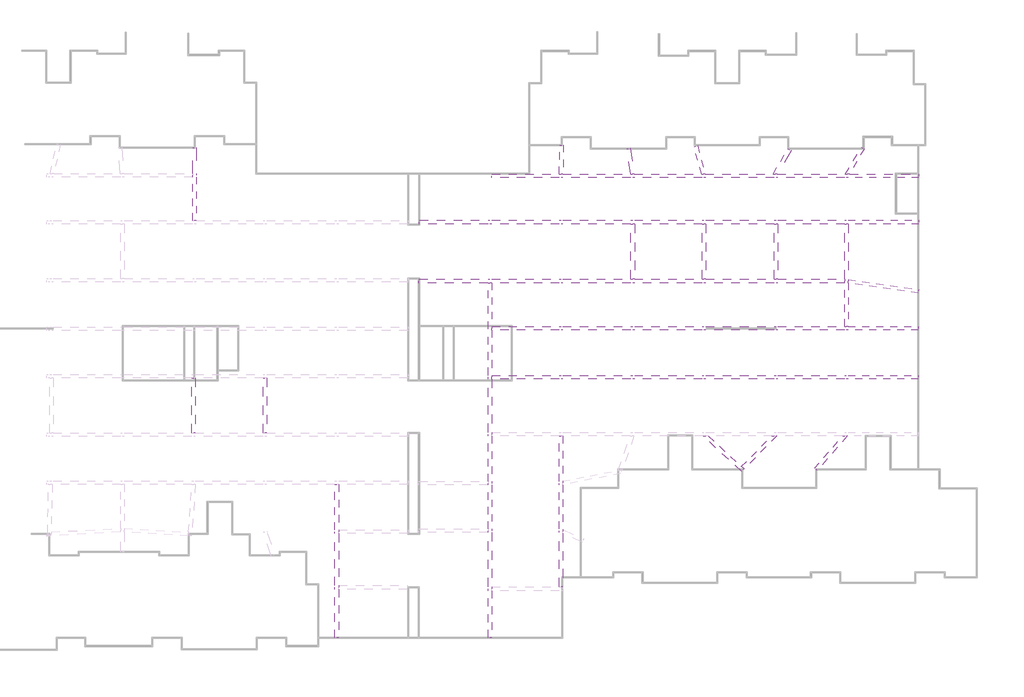
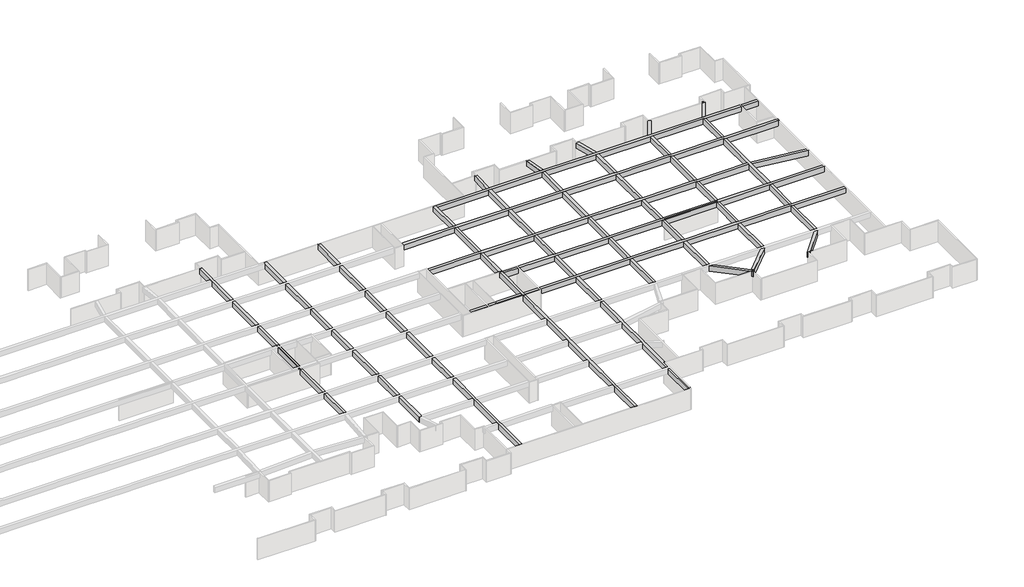
# One storey, part 16 of 16: 24 beams.
"""IFC4 building model written with IfcOpenShell, lengths in millimetres."""

from ifc_helpers import new_model, si_unit, frame, origin, place, context, project, spatial, polyline, outline, extrude, faceted_brep, element, save

model = new_model("IFC4")

# Units and contexts
model_context = context("Model", 3, world=origin())
ifc_project = project(units=[si_unit("LENGTHUNIT", "METRE", prefix="MILLI")], contexts=[model_context])

# Site, building, storey
site = spatial("IfcSite", under=ifc_project)
building = spatial("IfcBuilding", under=site)
storey = spatial("IfcBuildingStorey", under=building, Name="户型图", Elevation=0.0)

# Beams
placement = place(None, origin())
element("IfcBeam", 1, ObjectType="混凝土 - 矩形梁 : KL_beam", at=placement, inside=storey, context=model_context, shape_type="Brep", body=[
    faceted_brep([(470553.7576761, -137545.1471775, 3300.0), (470553.7576761, -137945.1471775, 3300.0), (470553.7576761, -137945.1471775, 2500.0), (470553.7576761, -137545.1471775, 2500.0), (414553.7576761, -137545.1471775, 3300.0), (414553.7576761, -137545.1471775, 2500.0), (414553.7576761, -137945.1471775, 2500.0), (414553.7576761, -137945.1471775, 3300.0), (462649.4319412, -137545.1471775, 3300.0), (462249.4319412, -137545.1471775, 3300.0), (454758.8748808, -137545.1471775, 3300.0), (454358.8748808, -137545.1471775, 3300.0), (446653.757676, -137545.1471775, 3300.0), (446253.757676, -137545.1471775, 3300.0), (438676.3481949, -137545.1471775, 3300.0), (438276.3481949, -137545.1471775, 3300.0), (430644.9716608, -137545.1471775, 3300.0), (430244.9716608, -137545.1471775, 3300.0), (422643.757676, -137545.1471775, 3300.0), (422243.757676, -137545.1471775, 3300.0), (422243.757676, -137945.1471775, 3300.0), (422643.757676, -137945.1471775, 3300.0), (430244.9716608, -137945.1471775, 3300.0), (430644.9716608, -137945.1471775, 3300.0), (438276.3481949, -137945.1471775, 3300.0), (438676.3481949, -137945.1471775, 3300.0), (446253.757676, -137945.1471775, 3300.0), (446653.757676, -137945.1471775, 3300.0), (454358.8748808, -137945.1471775, 3300.0), (454758.8748808, -137945.1471775, 3300.0), (462249.4319412, -137945.1471775, 3300.0), (462649.4319412, -137945.1471775, 3300.0), (422243.757676, -137945.1471775, 2500.0), (422643.757676, -137945.1471775, 2500.0), (430244.9716608, -137945.1471775, 2500.0), (430644.9716608, -137945.1471775, 2500.0), (438276.3481949, -137945.1471775, 2500.0), (438676.3481949, -137945.1471775, 2500.0), (446253.757676, -137945.1471775, 2500.0), (446653.757676, -137945.1471775, 2500.0), (454358.8748808, -137945.1471775, 2500.0), (454758.8748808, -137945.1471775, 2500.0), (462249.4319412, -137945.1471775, 2500.0), (462649.4319412, -137945.1471775, 2500.0), (422243.757676, -137545.1471775, 2500.0), (422643.757676, -137545.1471775, 2500.0), (430244.9716608, -137545.1471775, 2500.0), (430644.9716608, -137545.1471775, 2500.0), (438276.3481949, -137545.1471775, 2500.0), (438676.3481949, -137545.1471775, 2500.0), (446253.757676, -137545.1471775, 2500.0), (446653.757676, -137545.1471775, 2500.0), (454358.8748808, -137545.1471775, 2500.0), (454758.8748808, -137545.1471775, 2500.0), (462249.4319412, -137545.1471775, 2500.0), (462649.4319412, -137545.1471775, 2500.0)], [[[0, 1, 2, 3]], [[4, 5, 6, 7]], [[1, 0, 8, 9, 10, 11, 12, 13, 14, 15, 16, 17, 18, 19, 4, 7, 20, 21, 22, 23, 24, 25, 26, 27, 28, 29, 30, 31]], [[2, 1, 31, 30, 29, 28, 27, 26, 25, 24, 23, 22, 21, 20, 7, 6, 32, 33, 34, 35, 36, 37, 38, 39, 40, 41, 42, 43]], [[3, 2, 43, 42, 41, 40, 39, 38, 37, 36, 35, 34, 33, 32, 6, 5, 44, 45, 46, 47, 48, 49, 50, 51, 52, 53, 54, 55]], [[0, 3, 55, 54, 53, 52, 51, 50, 49, 48, 47, 46, 45, 44, 5, 4, 19, 18, 17, 16, 15, 14, 13, 12, 11, 10, 9, 8]]]),
])
element("IfcBeam", 2, ObjectType="混凝土 - 矩形梁 : KL_beam", at=placement, inside=storey, context=model_context, shape_type="Brep", body=[
    faceted_brep([(414504.0948086, -144165.1471774, 3300.0), (414504.0948086, -144165.1471774, 2500.0), (414504.0948086, -144565.1471774, 2500.0), (414504.0948086, -144565.1471774, 3300.0), (422243.757676, -144565.1471774, 3300.0), (422643.757676, -144565.1471774, 3300.0), (430244.9716608, -144565.1471774, 3300.0), (430644.9716608, -144565.1471774, 3300.0), (438276.3481949, -144565.1471774, 3300.0), (438676.3481949, -144565.1471774, 3300.0), (446253.757676, -144565.1471774, 3300.0), (446653.757676, -144565.1471774, 3300.0), (454358.8748808, -144565.1471774, 3300.0), (454758.8748808, -144565.1471774, 3300.0), (462249.4319412, -144565.1471774, 3300.0), (462249.4319412, -144165.1471774, 3300.0), (454758.8748808, -144165.1471774, 3300.0), (454358.8748808, -144165.1471774, 3300.0), (446653.757676, -144165.1471774, 3300.0), (446253.757676, -144165.1471774, 3300.0), (438676.3481949, -144165.1471774, 3300.0), (438276.3481949, -144165.1471774, 3300.0), (430644.9716608, -144165.1471774, 3300.0), (430244.9716608, -144165.1471774, 3300.0), (422643.757676, -144165.1471774, 3300.0), (422243.757676, -144165.1471774, 3300.0), (422243.757676, -144565.1471774, 2500.0), (422643.757676, -144565.1471774, 2500.0), (430244.9716608, -144565.1471774, 2500.0), (430644.9716608, -144565.1471774, 2500.0), (438276.3481949, -144565.1471774, 2500.0), (438676.3481949, -144565.1471774, 2500.0), (446253.757676, -144565.1471774, 2500.0), (446653.757676, -144565.1471774, 2500.0), (454358.8748808, -144565.1471774, 2500.0), (454758.8748808, -144565.1471774, 2500.0), (462249.4319412, -144565.1471774, 2500.0), (422243.757676, -144165.1471774, 2500.0), (422643.757676, -144165.1471774, 2500.0), (430244.9716608, -144165.1471774, 2500.0), (430644.9716608, -144165.1471774, 2500.0), (438276.3481949, -144165.1471774, 2500.0), (438676.3481949, -144165.1471774, 2500.0), (446253.757676, -144165.1471774, 2500.0), (446653.757676, -144165.1471774, 2500.0), (454358.8748808, -144165.1471774, 2500.0), (454758.8748808, -144165.1471774, 2500.0), (462249.4319412, -144165.1471774, 2500.0)], [[[0, 1, 2, 3]], [[0, 3, 4, 5, 6, 7, 8, 9, 10, 11, 12, 13, 14, 15, 16, 17, 18, 19, 20, 21, 22, 23, 24, 25]], [[3, 2, 26, 27, 28, 29, 30, 31, 32, 33, 34, 35, 36, 14, 13, 12, 11, 10, 9, 8, 7, 6, 5, 4]], [[2, 1, 37, 38, 39, 40, 41, 42, 43, 44, 45, 46, 47, 36, 35, 34, 33, 32, 31, 30, 29, 28, 27, 26]], [[1, 0, 25, 24, 23, 22, 21, 20, 19, 18, 17, 16, 15, 47, 46, 45, 44, 43, 42, 41, 40, 39, 38, 37]], [[15, 14, 36, 47]]]),
])
element("IfcBeam", 3, ObjectType="混凝土 - 矩形梁 : KL_beam", at=placement, inside=storey, context=model_context, shape_type="SweptSolid", body=[
    extrude(outline(polyline([(470533.1959149, -145291.6456152), (470477.5266745, -145687.7528427), (462649.4319412, -144587.5858748), (462649.4319412, -144183.6548458), (470533.1959149, -145291.6456152)])), frame((0.0, 0.0, 2500.0), z_axis=(0.0, 0.0, 1.0), x_axis=(1.0, 0.0, 0.0)), (0.0, 0.0, 1.0), 800.0),
])
element("IfcBeam", 4, ObjectType="混凝土 - 矩形梁 : KL_beam", at=placement, inside=storey, context=model_context, shape_type="Brep", body=[
    faceted_brep([(389113.757676, -129415.4343269, 3300.0), (389513.757676, -129415.4343269, 3300.0), (389513.757676, -129415.4343269, 2500.0), (389113.757676, -129415.4343269, 2500.0), (389113.757676, -132282.1518701, 3300.0), (389113.757676, -132682.1518701, 3300.0), (389113.757676, -137565.7214763, 3300.0), (389513.757676, -137565.7214763, 3300.0), (389513.757676, -132682.1518701, 3300.0), (389513.757676, -132282.1518701, 3300.0), (389513.757676, -137565.7214763, 2500.0), (389513.757676, -132682.1518701, 2500.0), (389513.757676, -132282.1518701, 2500.0), (389113.757676, -137565.7214763, 2500.0), (389113.757676, -132682.1518701, 2500.0), (389113.757676, -132282.1518701, 2500.0)], [[[0, 1, 2, 3]], [[1, 0, 4, 5, 6, 7, 8, 9]], [[2, 1, 9, 8, 7, 10, 11, 12]], [[3, 2, 12, 11, 10, 13, 14, 15]], [[0, 3, 15, 14, 13, 6, 5, 4]], [[7, 6, 13, 10]]]),
    faceted_brep([(389513.757676, -149515.4343269, 3300.0), (389113.757676, -149515.4343269, 3300.0), (389113.757676, -149515.4343269, 2500.0), (389513.757676, -149515.4343269, 2500.0), (389113.757676, -144485.7214763, 3300.0), (389513.757676, -144485.7214763, 3300.0), (389513.757676, -144485.7214763, 2500.0), (389113.757676, -144485.7214763, 2500.0)], [[[0, 1, 2, 3]], [[4, 5, 6, 7]], [[1, 0, 5, 4]], [[0, 3, 6, 5]], [[3, 2, 7, 6]], [[2, 1, 4, 7]]]),
    faceted_brep([(389113.757676, -137965.7214763, 3300.0), (389513.757676, -137965.7214763, 3300.0), (389513.757676, -137965.7214763, 2500.0), (389113.757676, -137965.7214763, 2500.0), (389113.757676, -144085.7214763, 3300.0), (389513.757676, -144085.7214763, 3300.0), (389513.757676, -144085.7214763, 2500.0), (389113.757676, -144085.7214763, 2500.0)], [[[0, 1, 2, 3]], [[1, 0, 4, 5]], [[2, 1, 5, 6]], [[3, 2, 6, 7]], [[0, 3, 7, 4]], [[5, 4, 7, 6]]]),
])
element("IfcBeam", 5, ObjectType="混凝土 - 矩形梁 : KL_beam", at=placement, inside=storey, context=model_context, shape_type="Brep", body=[
    faceted_brep([(397025.7298502, -137565.7214763, 3300.0), (397425.7298502, -137565.7214763, 3300.0), (397425.7298502, -132282.1518701, 3300.0), (397025.7298502, -132282.1518701, 3300.0), (397025.7298502, -132682.1518701, 3300.0), (397025.7298502, -137565.7214763, 2500.0), (397025.7298502, -132282.1518701, 2500.0), (397025.7298502, -132682.1518701, 2500.0), (397425.7298502, -137565.7214763, 2500.0), (397425.7298502, -132282.1518701, 2500.0)], [[[0, 1, 2, 3, 4]], [[5, 0, 4, 3, 6, 7]], [[8, 5, 7, 6, 9]], [[1, 8, 9, 2]], [[1, 0, 5, 8]], [[3, 2, 9, 6]]]),
    faceted_brep([(397025.7298502, -137965.7214763, 3300.0), (397425.7298502, -137965.7214763, 3300.0), (397425.7298502, -137965.7214763, 2500.0), (397025.7298502, -137965.7214763, 2500.0), (397425.7298502, -144085.7214763, 3300.0), (397025.7298502, -144085.7214763, 3300.0), (397025.7298502, -144085.7214763, 2500.0), (397425.7298502, -144085.7214763, 2500.0)], [[[0, 1, 2, 3]], [[4, 5, 6, 7]], [[1, 0, 5, 4]], [[0, 3, 6, 5]], [[3, 2, 7, 6]], [[2, 1, 4, 7]]]),
    faceted_brep([(397425.7298502, -149515.4343269, 3300.0), (397425.7298502, -144485.7214763, 3300.0), (397025.7298502, -144485.7214763, 3300.0), (397025.7298502, -149515.4343269, 3300.0), (397025.7298502, -144485.7214763, 2500.0), (397025.7298502, -149515.4343269, 2500.0), (397425.7298502, -144485.7214763, 2500.0), (397425.7298502, -149515.4343269, 2500.0)], [[[0, 1, 2, 3]], [[3, 2, 4, 5]], [[5, 4, 6, 7]], [[1, 0, 7, 6]], [[2, 1, 6, 4]], [[0, 3, 5, 7]]]),
    faceted_brep([(397025.7298502, -149915.4343269, 3300.0), (397425.7298502, -149915.4343269, 3300.0), (397425.7298502, -149915.4343269, 2500.0), (397025.7298502, -149915.4343269, 2500.0), (397425.7298502, -154845.1471774, 3300.0), (397025.7298502, -154845.1471774, 3300.0), (397025.7298502, -154845.1471774, 2500.0), (397425.7298502, -154845.1471774, 2500.0)], [[[0, 1, 2, 3]], [[4, 5, 6, 7]], [[4, 1, 0, 5]], [[5, 0, 3, 6]], [[6, 3, 2, 7]], [[1, 4, 7, 2]]]),
    faceted_brep([(397025.7298502, -155245.1471774, 3300.0), (397425.7298502, -155245.1471774, 3300.0), (397425.7298502, -155245.1471774, 2500.0), (397025.7298502, -155245.1471774, 2500.0), (397425.7298502, -161426.0461868, 3300.0), (397025.7298502, -161426.0461868, 3300.0), (397025.7298502, -161426.0461868, 2500.0), (397425.7298502, -161426.0461868, 2500.0)], [[[0, 1, 2, 3]], [[4, 5, 6, 7]], [[4, 1, 0, 5]], [[5, 0, 3, 6]], [[6, 3, 2, 7]], [[1, 4, 7, 2]]]),
    faceted_brep([(397025.7298502, -161826.0461868, 3300.0), (397425.7298502, -161826.0461868, 3300.0), (397425.7298502, -161826.0461868, 2500.0), (397025.7298502, -161826.0461868, 2500.0), (397425.7298502, -166805.1471774, 3300.0), (397025.7298502, -166805.1471774, 3300.0), (397025.7298502, -166805.1471774, 2500.0), (397425.7298502, -166805.1471774, 2500.0)], [[[0, 1, 2, 3]], [[4, 5, 6, 7]], [[1, 0, 5, 4]], [[0, 3, 6, 5]], [[3, 2, 7, 6]], [[2, 1, 4, 7]]]),
    faceted_brep([(397025.7298502, -167205.1471774, 3300.0), (397425.7298502, -167205.1471774, 3300.0), (397425.7298502, -167205.1471774, 2500.0), (397025.7298502, -167205.1471774, 2500.0), (397425.7298502, -172471.6786556, 3300.0), (397025.7298502, -172538.6156993, 3300.0), (397025.7298502, -172538.6156993, 2500.0), (397425.7298502, -172471.6786556, 2500.0), (397425.7298502, -172305.1471775, 3300.0), (397425.7298502, -172305.1471775, 2500.0)], [[[0, 1, 2, 3]], [[4, 5, 6, 7]], [[5, 4, 8, 1, 0]], [[6, 5, 0, 3]], [[7, 6, 3, 2, 9]], [[4, 7, 9, 2, 1, 8]]]),
])
element("IfcBeam", 6, ObjectType="混凝土 - 矩形梁 : KL_beam", at=placement, inside=storey, context=model_context, shape_type="Brep", body=[
    faceted_brep([(405478.7576761, -184405.1471774, 3300.0), (405078.7576761, -184405.1471774, 3300.0), (405078.7576761, -184405.1471774, 2500.0), (405478.7576761, -184405.1471774, 2500.0), (405478.7576761, -178936.89075, 3300.0), (405478.7576761, -178536.89075, 3300.0), (405478.7576761, -172705.1471775, 3300.0), (405478.7576761, -172305.1471775, 3300.0), (405478.7576761, -167205.1471774, 3300.0), (405078.7576761, -167205.1471774, 3300.0), (405078.7576761, -172305.1471775, 3300.0), (405078.7576761, -172705.1471775, 3300.0), (405078.7576761, -178536.89075, 3300.0), (405078.7576761, -178936.89075, 3300.0), (405078.7576761, -167205.1471774, 2500.0), (405078.7576761, -172305.1471775, 2500.0), (405078.7576761, -172705.1471775, 2500.0), (405078.7576761, -178536.89075, 2500.0), (405078.7576761, -178936.89075, 2500.0), (405478.7576761, -167205.1471774, 2500.0), (405478.7576761, -172305.1471775, 2500.0), (405478.7576761, -172705.1471775, 2500.0), (405478.7576761, -178536.89075, 2500.0), (405478.7576761, -178936.89075, 2500.0)], [[[0, 1, 2, 3]], [[1, 0, 4, 5, 6, 7, 8, 9, 10, 11, 12, 13]], [[2, 1, 13, 12, 11, 10, 9, 14, 15, 16, 17, 18]], [[3, 2, 18, 17, 16, 15, 14, 19, 20, 21, 22, 23]], [[0, 3, 23, 22, 21, 20, 19, 8, 7, 6, 5, 4]], [[9, 8, 19, 14]]]),
    faceted_brep([(405478.7576761, -132305.1471774, 3300.0), (405478.7576761, -132305.1471774, 2500.0), (405078.7576761, -132305.1471774, 2500.0), (405078.7576761, -132305.1471774, 3300.0), (405478.7576761, -137565.7214763, 3300.0), (405078.7576761, -137565.7214763, 3300.0), (405078.7576761, -137565.7214763, 2500.0), (405478.7576761, -137565.7214763, 2500.0)], [[[0, 1, 2, 3]], [[4, 5, 6, 7]], [[0, 3, 5, 4]], [[3, 2, 6, 5]], [[2, 1, 7, 6]], [[1, 0, 4, 7]]]),
    faceted_brep([(405078.7576761, -137965.7214763, 3300.0), (405478.7576761, -137965.7214763, 3300.0), (405478.7576761, -137965.7214763, 2500.0), (405078.7576761, -137965.7214763, 2500.0), (405478.7576761, -144085.7214763, 3300.0), (405078.7576761, -144085.7214763, 3300.0), (405078.7576761, -144085.7214763, 2500.0), (405478.7576761, -144085.7214763, 2500.0)], [[[0, 1, 2, 3]], [[4, 5, 6, 7]], [[1, 0, 5, 4]], [[0, 3, 6, 5]], [[3, 2, 7, 6]], [[2, 1, 4, 7]]]),
    faceted_brep([(405078.7576761, -144485.7214763, 3300.0), (405478.7576761, -144485.7214763, 3300.0), (405478.7576761, -144485.7214763, 2500.0), (405078.7576761, -144485.7214763, 2500.0), (405478.7576761, -149515.4343269, 3300.0), (405078.7576761, -149515.4343269, 3300.0), (405078.7576761, -149515.4343269, 2500.0), (405478.7576761, -149515.4343269, 2500.0)], [[[0, 1, 2, 3]], [[4, 5, 6, 7]], [[1, 0, 5, 4]], [[0, 3, 6, 5]], [[3, 2, 7, 6]], [[2, 1, 4, 7]]]),
    faceted_brep([(405078.7576761, -149915.4343269, 3300.0), (405478.7576761, -149915.4343269, 3300.0), (405478.7576761, -149915.4343269, 2500.0), (405078.7576761, -149915.4343269, 2500.0), (405478.7576761, -154845.1471774, 3300.0), (405078.7576761, -154845.1471774, 3300.0), (405078.7576761, -154845.1471774, 2500.0), (405478.7576761, -154845.1471774, 2500.0)], [[[0, 1, 2, 3]], [[4, 5, 6, 7]], [[1, 0, 5, 4]], [[0, 3, 6, 5]], [[3, 2, 7, 6]], [[2, 1, 4, 7]]]),
    faceted_brep([(405078.7576761, -155245.1471774, 3300.0), (405478.7576761, -155245.1471774, 3300.0), (405478.7576761, -155245.1471774, 2500.0), (405078.7576761, -155245.1471774, 2500.0), (405478.7576761, -161426.0461868, 3300.0), (405078.7576761, -161426.0461868, 3300.0), (405078.7576761, -161426.0461868, 2500.0), (405478.7576761, -161426.0461868, 2500.0)], [[[0, 1, 2, 3]], [[4, 5, 6, 7]], [[1, 0, 5, 4]], [[0, 3, 6, 5]], [[3, 2, 7, 6]], [[2, 1, 4, 7]]]),
    faceted_brep([(405078.7576761, -161826.0461868, 3300.0), (405478.7576761, -161826.0461868, 3300.0), (405478.7576761, -161826.0461868, 2500.0), (405078.7576761, -161826.0461868, 2500.0), (405478.7576761, -166805.1471774, 3300.0), (405078.7576761, -166805.1471774, 3300.0), (405078.7576761, -166805.1471774, 2500.0), (405478.7576761, -166805.1471774, 2500.0)], [[[0, 1, 2, 3]], [[4, 5, 6, 7]], [[1, 0, 5, 4]], [[0, 3, 6, 5]], [[3, 2, 7, 6]], [[2, 1, 4, 7]]]),
])
element("IfcBeam", 7, ObjectType="混凝土 - 矩形梁 : KL_beam", at=placement, inside=storey, context=model_context, shape_type="SweptSolid", body=[
    extrude(outline(polyline([(389433.5747738, -166805.1471774), (389033.5747738, -166805.1471774), (389033.5747738, -161826.0461868), (389433.5747738, -161826.0461868), (389433.5747738, -166805.1471774)])), frame((0.0, 0.0, 2500.0), z_axis=(0.0, 0.0, 1.0), x_axis=(1.0, 0.0, 0.0)), (0.0, 0.0, 1.0), 800.0),
    extrude(outline(polyline([(389033.5747738, -149915.4343269), (389433.5747738, -149915.4343269), (389433.5747738, -154845.1471774), (389033.5747738, -154845.1471774), (389033.5747738, -149915.4343269)])), frame((0.0, 0.0, 2500.0), z_axis=(0.0, 0.0, 1.0), x_axis=(1.0, 0.0, 0.0)), (0.0, 0.0, 1.0), 800.0),
    extrude(outline(polyline([(389033.5747738, -155245.1471774), (389433.5747738, -155245.1471774), (389433.5747738, -161426.0461868), (389033.5747738, -161426.0461868), (389033.5747738, -155245.1471774)])), frame((0.0, 0.0, 2500.0), z_axis=(0.0, 0.0, 1.0), x_axis=(1.0, 0.0, 0.0)), (0.0, 0.0, 1.0), 800.0),
])
element("IfcBeam", 8, ObjectType="混凝土 - 矩形梁 : KL_beam", at=placement, inside=storey, context=model_context, shape_type="Brep", body=[
    faceted_brep([(422643.757676, -184405.1471774, 3300.0), (422243.757676, -184405.1471774, 3300.0), (422243.757676, -184405.1471774, 2500.0), (422643.757676, -184405.1471774, 2500.0), (422643.757676, -179105.1471774, 3300.0), (422643.757676, -178705.1471774, 3300.0), (422643.757676, -172582.0297951, 3300.0), (422643.757676, -172182.0297951, 3300.0), (422643.757676, -167272.0227911, 3300.0), (422643.757676, -166872.0227911, 3300.0), (422643.757676, -161762.0157871, 3300.0), (422643.757676, -161362.0157871, 3300.0), (422643.757676, -155345.1471774, 3300.0), (422643.757676, -154945.1471774, 3300.0), (422643.757676, -149865.1471775, 3300.0), (422643.757676, -149465.1471775, 3300.0), (422643.757676, -144565.1471774, 3300.0), (422243.757676, -144565.1471774, 3300.0), (422243.757676, -154945.1471774, 3300.0), (422243.757676, -155345.1471774, 3300.0), (422243.757676, -161362.0157871, 3300.0), (422243.757676, -161762.0157871, 3300.0), (422243.757676, -166872.0227911, 3300.0), (422243.757676, -167272.0227911, 3300.0), (422243.757676, -172182.0297951, 3300.0), (422243.757676, -172582.0297951, 3300.0), (422243.757676, -178705.1471774, 3300.0), (422243.757676, -179105.1471774, 3300.0), (422243.757676, -144565.1471774, 2500.0), (422243.757676, -154945.1471774, 2500.0), (422243.757676, -155345.1471774, 2500.0), (422243.757676, -161362.0157871, 2500.0), (422243.757676, -161762.0157871, 2500.0), (422243.757676, -166872.0227911, 2500.0), (422243.757676, -167272.0227911, 2500.0), (422243.757676, -172182.0297951, 2500.0), (422243.757676, -172582.0297951, 2500.0), (422243.757676, -178705.1471774, 2500.0), (422243.757676, -179105.1471774, 2500.0), (422643.757676, -144565.1471774, 2500.0), (422643.757676, -149465.1471775, 2500.0), (422643.757676, -149865.1471775, 2500.0), (422643.757676, -154945.1471774, 2500.0), (422643.757676, -155345.1471774, 2500.0), (422643.757676, -161362.0157871, 2500.0), (422643.757676, -161762.0157871, 2500.0), (422643.757676, -166872.0227911, 2500.0), (422643.757676, -167272.0227911, 2500.0), (422643.757676, -172182.0297951, 2500.0), (422643.757676, -172582.0297951, 2500.0), (422643.757676, -178705.1471774, 2500.0), (422643.757676, -179105.1471774, 2500.0)], [[[0, 1, 2, 3]], [[1, 0, 4, 5, 6, 7, 8, 9, 10, 11, 12, 13, 14, 15, 16, 17, 18, 19, 20, 21, 22, 23, 24, 25, 26, 27]], [[2, 1, 27, 26, 25, 24, 23, 22, 21, 20, 19, 18, 17, 28, 29, 30, 31, 32, 33, 34, 35, 36, 37, 38]], [[3, 2, 38, 37, 36, 35, 34, 33, 32, 31, 30, 29, 28, 39, 40, 41, 42, 43, 44, 45, 46, 47, 48, 49, 50, 51]], [[0, 3, 51, 50, 49, 48, 47, 46, 45, 44, 43, 42, 41, 40, 39, 16, 15, 14, 13, 12, 11, 10, 9, 8, 7, 6, 5, 4]], [[17, 16, 39, 28]]]),
    faceted_brep([(422643.757676, -132305.1471774, 3300.0), (422643.757676, -132305.1471774, 2500.0), (422243.757676, -132305.1471774, 2500.0), (422243.757676, -132305.1471774, 3300.0), (422643.757676, -137545.1471775, 3300.0), (422243.757676, -137545.1471775, 3300.0), (422243.757676, -137545.1471775, 2500.0), (422643.757676, -137545.1471775, 2500.0), (422643.757676, -132765.1471775, 3300.0), (422643.757676, -132365.1471775, 3300.0), (422643.757676, -132365.1471775, 2500.0), (422643.757676, -132765.1471775, 2500.0)], [[[0, 1, 2, 3]], [[4, 5, 6, 7]], [[0, 3, 5, 4, 8, 9]], [[3, 2, 6, 5]], [[2, 1, 10, 11, 7, 6]], [[1, 0, 9, 8, 4, 7, 11, 10]]]),
    faceted_brep([(422243.757676, -137945.1471775, 3300.0), (422643.757676, -137945.1471775, 3300.0), (422643.757676, -137945.1471775, 2500.0), (422243.757676, -137945.1471775, 2500.0), (422643.757676, -144165.1471774, 3300.0), (422243.757676, -144165.1471774, 3300.0), (422243.757676, -144165.1471774, 2500.0), (422643.757676, -144165.1471774, 2500.0)], [[[0, 1, 2, 3]], [[4, 5, 6, 7]], [[1, 0, 5, 4]], [[0, 3, 6, 5]], [[3, 2, 7, 6]], [[2, 1, 4, 7]]]),
])
element("IfcBeam", 9, ObjectType="混凝土 - 矩形梁 : KL_beam", at=placement, inside=storey, context=model_context, shape_type="Brep", body=[
    faceted_brep([(470505.1087926, -154945.1471774, 3300.0), (470505.1087926, -155345.1471774, 3300.0), (470505.1087926, -155345.1471774, 2500.0), (470505.1087926, -154945.1471774, 2500.0), (462649.4319412, -154945.1471774, 3300.0), (462249.4319412, -154945.1471774, 3300.0), (454758.8748808, -154945.1471774, 3300.0), (454358.8748808, -154945.1471774, 3300.0), (446653.757676, -154945.1471774, 3300.0), (446253.757676, -154945.1471774, 3300.0), (438676.3481949, -154945.1471774, 3300.0), (438276.3481949, -154945.1471774, 3300.0), (430644.9716608, -154945.1471774, 3300.0), (430244.9716608, -154945.1471774, 3300.0), (422643.757676, -154945.1471774, 3300.0), (422643.757676, -155345.1471774, 3300.0), (430244.9716608, -155345.1471774, 3300.0), (430644.9716608, -155345.1471774, 3300.0), (438276.3481949, -155345.1471774, 3300.0), (438676.3481949, -155345.1471774, 3300.0), (446253.757676, -155345.1471774, 3300.0), (446653.757676, -155345.1471774, 3300.0), (454358.8748808, -155345.1471774, 3300.0), (454758.8748808, -155345.1471774, 3300.0), (462249.4319412, -155345.1471774, 3300.0), (462649.4319412, -155345.1471774, 3300.0), (422643.757676, -155345.1471774, 2500.0), (430244.9716608, -155345.1471774, 2500.0), (430644.9716608, -155345.1471774, 2500.0), (438276.3481949, -155345.1471774, 2500.0), (438676.3481949, -155345.1471774, 2500.0), (446253.757676, -155345.1471774, 2500.0), (446653.757676, -155345.1471774, 2500.0), (454358.8748808, -155345.1471774, 2500.0), (454758.8748808, -155345.1471774, 2500.0), (462249.4319412, -155345.1471774, 2500.0), (462649.4319412, -155345.1471774, 2500.0), (422643.757676, -154945.1471774, 2500.0), (430244.9716608, -154945.1471774, 2500.0), (430644.9716608, -154945.1471774, 2500.0), (438276.3481949, -154945.1471774, 2500.0), (438676.3481949, -154945.1471774, 2500.0), (446253.757676, -154945.1471774, 2500.0), (446653.757676, -154945.1471774, 2500.0), (454358.8748808, -154945.1471774, 2500.0), (454758.8748808, -154945.1471774, 2500.0), (462249.4319412, -154945.1471774, 2500.0), (462649.4319412, -154945.1471774, 2500.0)], [[[0, 1, 2, 3]], [[1, 0, 4, 5, 6, 7, 8, 9, 10, 11, 12, 13, 14, 15, 16, 17, 18, 19, 20, 21, 22, 23, 24, 25]], [[2, 1, 25, 24, 23, 22, 21, 20, 19, 18, 17, 16, 15, 26, 27, 28, 29, 30, 31, 32, 33, 34, 35, 36]], [[3, 2, 36, 35, 34, 33, 32, 31, 30, 29, 28, 27, 26, 37, 38, 39, 40, 41, 42, 43, 44, 45, 46, 47]], [[0, 3, 47, 46, 45, 44, 43, 42, 41, 40, 39, 38, 37, 14, 13, 12, 11, 10, 9, 8, 7, 6, 5, 4]], [[15, 14, 37, 26]]]),
    faceted_brep([(414504.1087926, -154945.1471774, 3300.0), (414504.1087926, -154945.1471774, 2500.0), (414504.1087926, -155345.1471774, 2500.0), (414504.1087926, -155345.1471774, 3300.0), (422243.757676, -154945.1471774, 3300.0), (422243.757676, -155345.1471774, 3300.0), (422243.757676, -155345.1471774, 2500.0), (422243.757676, -154945.1471774, 2500.0)], [[[0, 1, 2, 3]], [[4, 5, 6, 7]], [[0, 3, 5, 4]], [[3, 2, 6, 5]], [[2, 1, 7, 6]], [[1, 0, 4, 7]]]),
])
element("IfcBeam", 10, ObjectType="混凝土 - 矩形梁 : KL_beam", at=placement, inside=storey, context=model_context, shape_type="Brep", body=[
    faceted_brep([(470505.1087925, -149465.1471775, 3300.0), (470505.1087925, -149865.1471775, 3300.0), (470505.1087925, -149865.1471775, 2500.0), (470505.1087925, -149465.1471775, 2500.0), (462649.4319412, -149465.1471775, 3300.0), (462249.4319412, -149465.1471775, 3300.0), (454758.8748808, -149465.1471775, 3300.0), (454358.8748808, -149465.1471775, 3300.0), (446653.757676, -149465.1471775, 3300.0), (446253.757676, -149465.1471775, 3300.0), (438676.3481949, -149465.1471775, 3300.0), (438276.3481949, -149465.1471775, 3300.0), (430644.9716608, -149465.1471775, 3300.0), (430244.9716608, -149465.1471775, 3300.0), (422643.757676, -149465.1471775, 3300.0), (422643.757676, -149865.1471775, 3300.0), (430244.9716608, -149865.1471775, 3300.0), (430644.9716608, -149865.1471775, 3300.0), (438276.3481949, -149865.1471775, 3300.0), (438676.3481949, -149865.1471775, 3300.0), (446253.757676, -149865.1471775, 3300.0), (446653.757676, -149865.1471775, 3300.0), (454358.8748808, -149865.1471775, 3300.0), (454758.8748808, -149865.1471775, 3300.0), (462249.4319412, -149865.1471775, 3300.0), (462649.4319412, -149865.1471775, 3300.0), (422643.757676, -149865.1471775, 2500.0), (430244.9716608, -149865.1471775, 2500.0), (430644.9716608, -149865.1471775, 2500.0), (438276.3481949, -149865.1471775, 2500.0), (438676.3481949, -149865.1471775, 2500.0), (446253.757676, -149865.1471775, 2500.0), (446653.757676, -149865.1471775, 2500.0), (454358.8748808, -149865.1471775, 2500.0), (454758.8748808, -149865.1471775, 2500.0), (462249.4319412, -149865.1471775, 2500.0), (462649.4319412, -149865.1471775, 2500.0), (422643.757676, -149465.1471775, 2500.0), (430244.9716608, -149465.1471775, 2500.0), (430644.9716608, -149465.1471775, 2500.0), (438276.3481949, -149465.1471775, 2500.0), (438676.3481949, -149465.1471775, 2500.0), (446253.757676, -149465.1471775, 2500.0), (446653.757676, -149465.1471775, 2500.0), (454358.8748808, -149465.1471775, 2500.0), (454758.8748808, -149465.1471775, 2500.0), (462249.4319412, -149465.1471775, 2500.0), (462649.4319412, -149465.1471775, 2500.0)], [[[0, 1, 2, 3]], [[1, 0, 4, 5, 6, 7, 8, 9, 10, 11, 12, 13, 14, 15, 16, 17, 18, 19, 20, 21, 22, 23, 24, 25]], [[2, 1, 25, 24, 23, 22, 21, 20, 19, 18, 17, 16, 15, 26, 27, 28, 29, 30, 31, 32, 33, 34, 35, 36]], [[3, 2, 36, 35, 34, 33, 32, 31, 30, 29, 28, 27, 26, 37, 38, 39, 40, 41, 42, 43, 44, 45, 46, 47]], [[0, 3, 47, 46, 45, 44, 43, 42, 41, 40, 39, 38, 37, 14, 13, 12, 11, 10, 9, 8, 7, 6, 5, 4]], [[15, 14, 37, 26]]]),
])
element("IfcBeam", 11, ObjectType="混凝土 - 矩形梁 : KL_beam", at=placement, inside=storey, context=model_context, shape_type="Brep", body=[
    faceted_brep([(470543.757676, -132365.1471775, 3300.0), (470543.757676, -132765.1471775, 3300.0), (470543.757676, -132765.1471775, 2500.0), (470543.757676, -132365.1471775, 2500.0), (462795.8421027, -132365.1471775, 3300.0), (462333.9618873, -132365.1471775, 3300.0), (454705.2850424, -132365.1471775, 3300.0), (454243.404827, -132365.1471775, 3300.0), (446607.2230736, -132365.1471775, 3300.0), (446193.1126015, -132365.1471775, 3300.0), (438647.164332, -132365.1471775, 3300.0), (438242.1782817, -132365.1471775, 3300.0), (430648.4931394, -132365.1471775, 3300.0), (430248.4322082, -132365.1471775, 3300.0), (422643.757676, -132365.1471775, 3300.0), (422643.757676, -132765.1471775, 3300.0), (430244.9716608, -132765.1471775, 3300.0), (430644.9716608, -132765.1471775, 3300.0), (438276.3481949, -132765.1471775, 3300.0), (438676.3481949, -132765.1471775, 3300.0), (446253.757676, -132765.1471775, 3300.0), (446653.757676, -132765.1471775, 3300.0), (454358.8748808, -132765.1471775, 3300.0), (454758.8748808, -132765.1471775, 3300.0), (462249.4319412, -132765.1471775, 3300.0), (462649.4319412, -132765.1471775, 3300.0), (422643.757676, -132765.1471775, 2500.0), (430244.9716608, -132765.1471775, 2500.0), (430644.9716608, -132765.1471775, 2500.0), (438276.3481949, -132765.1471775, 2500.0), (438676.3481949, -132765.1471775, 2500.0), (446253.757676, -132765.1471775, 2500.0), (446653.757676, -132765.1471775, 2500.0), (454358.8748808, -132765.1471775, 2500.0), (454758.8748808, -132765.1471775, 2500.0), (462249.4319412, -132765.1471775, 2500.0), (462649.4319412, -132765.1471775, 2500.0), (422643.757676, -132365.1471775, 2500.0), (430248.4322082, -132365.1471775, 2500.0), (430648.4931394, -132365.1471775, 2500.0), (438242.1782817, -132365.1471775, 2500.0), (438647.164332, -132365.1471775, 2500.0), (446193.1126015, -132365.1471775, 2500.0), (446607.2230736, -132365.1471775, 2500.0), (454243.404827, -132365.1471775, 2500.0), (454705.2850424, -132365.1471775, 2500.0), (462333.9618873, -132365.1471775, 2500.0), (462795.8421027, -132365.1471775, 2500.0)], [[[0, 1, 2, 3]], [[1, 0, 4, 5, 6, 7, 8, 9, 10, 11, 12, 13, 14, 15, 16, 17, 18, 19, 20, 21, 22, 23, 24, 25]], [[2, 1, 25, 24, 23, 22, 21, 20, 19, 18, 17, 16, 15, 26, 27, 28, 29, 30, 31, 32, 33, 34, 35, 36]], [[3, 2, 36, 35, 34, 33, 32, 31, 30, 29, 28, 27, 26, 37, 38, 39, 40, 41, 42, 43, 44, 45, 46, 47]], [[0, 3, 47, 46, 45, 44, 43, 42, 41, 40, 39, 38, 37, 14, 13, 12, 11, 10, 9, 8, 7, 6, 5, 4]], [[15, 14, 37, 26]]]),
])
element("IfcBeam", 12, ObjectType="混凝土 - 矩形梁 : KL_beam", at=placement, inside=storey, context=model_context, shape_type="SweptSolid", body=[
    extrude(outline(polyline([(430305.4306647, -129099.7077893), (430705.3697428, -129106.6887518), (430648.4931394, -132365.1471775), (430248.4322082, -132365.1471775), (430305.4306647, -129099.7077893)])), frame((0.0, 0.0, 2500.0), z_axis=(0.0, 0.0, 1.0), x_axis=(1.0, 0.0, 0.0)), (0.0, 0.0, 1.0), 800.0),
])
element("IfcBeam", 13, ObjectType="混凝土 - 矩形梁 : KL_beam", at=placement, inside=storey, context=model_context, shape_type="Brep", body=[
    faceted_brep([(430644.9716608, -184165.1471775, 3300.0), (430244.9716608, -184165.1471775, 3300.0), (430244.9716608, -184165.1471775, 2500.0), (430644.9716608, -184165.1471775, 2500.0), (430644.9716608, -179105.1471774, 3300.0), (430244.9716608, -179105.1471774, 3300.0), (430244.9716608, -179105.1471774, 2500.0), (430644.9716608, -179105.1471774, 2500.0)], [[[0, 1, 2, 3]], [[1, 0, 4, 5]], [[2, 1, 5, 6]], [[3, 2, 6, 7]], [[0, 3, 7, 4]], [[5, 4, 7, 6]]]),
    faceted_brep([(430244.9716608, -132765.1471775, 3300.0), (430644.9716608, -132765.1471775, 3300.0), (430644.9716608, -132765.1471775, 2500.0), (430244.9716608, -132765.1471775, 2500.0), (430644.9716608, -137545.1471775, 3300.0), (430244.9716608, -137545.1471775, 3300.0), (430244.9716608, -137545.1471775, 2500.0), (430644.9716608, -137545.1471775, 2500.0)], [[[0, 1, 2, 3]], [[4, 5, 6, 7]], [[1, 0, 5, 4]], [[0, 3, 6, 5]], [[3, 2, 7, 6]], [[2, 1, 4, 7]]]),
    faceted_brep([(430244.9716608, -137945.1471775, 3300.0), (430644.9716608, -137945.1471775, 3300.0), (430644.9716608, -137945.1471775, 2500.0), (430244.9716608, -137945.1471775, 2500.0), (430644.9716608, -144165.1471774, 3300.0), (430244.9716608, -144165.1471774, 3300.0), (430244.9716608, -144165.1471774, 2500.0), (430644.9716608, -144165.1471774, 2500.0)], [[[0, 1, 2, 3]], [[4, 5, 6, 7]], [[1, 0, 5, 4]], [[0, 3, 6, 5]], [[3, 2, 7, 6]], [[2, 1, 4, 7]]]),
    faceted_brep([(430244.9716608, -144565.1471774, 3300.0), (430644.9716608, -144565.1471774, 3300.0), (430644.9716608, -144565.1471774, 2500.0), (430244.9716608, -144565.1471774, 2500.0), (430644.9716608, -149465.1471775, 3300.0), (430244.9716608, -149465.1471775, 3300.0), (430244.9716608, -149465.1471775, 2500.0), (430644.9716608, -149465.1471775, 2500.0)], [[[0, 1, 2, 3]], [[4, 5, 6, 7]], [[1, 0, 5, 4]], [[0, 3, 6, 5]], [[3, 2, 7, 6]], [[2, 1, 4, 7]]]),
    faceted_brep([(430644.9716608, -178705.1471774, 3300.0), (430244.9716608, -178705.1471774, 3300.0), (430244.9716608, -178705.1471774, 2500.0), (430644.9716608, -178705.1471774, 2500.0), (430644.9716608, -172668.5545414, 3300.0), (430644.9716608, -172227.2033738, 3300.0), (430644.9716608, -167228.8788811, 3300.0), (430644.9716608, -166821.3922032, 3300.0), (430644.9716608, -161762.0157871, 3300.0), (430244.9716608, -161762.0157871, 3300.0), (430244.9716608, -166872.0227911, 3300.0), (430244.9716608, -167272.0227911, 3300.0), (430244.9716608, -172182.0297951, 3300.0), (430244.9716608, -172582.0297951, 3300.0), (430244.9716608, -161762.0157871, 2500.0), (430244.9716608, -166872.0227911, 2500.0), (430244.9716608, -167272.0227911, 2500.0), (430244.9716608, -172182.0297951, 2500.0), (430244.9716608, -172582.0297951, 2500.0), (430644.9716608, -161762.0157871, 2500.0), (430644.9716608, -166821.3922032, 2500.0), (430644.9716608, -167228.8788811, 2500.0), (430644.9716608, -172227.2033738, 2500.0), (430644.9716608, -172668.5545414, 2500.0)], [[[0, 1, 2, 3]], [[1, 0, 4, 5, 6, 7, 8, 9, 10, 11, 12, 13]], [[2, 1, 13, 12, 11, 10, 9, 14, 15, 16, 17, 18]], [[3, 2, 18, 17, 16, 15, 14, 19, 20, 21, 22, 23]], [[0, 3, 23, 22, 21, 20, 19, 8, 7, 6, 5, 4]], [[9, 8, 19, 14]]]),
    faceted_brep([(430644.9716608, -161362.0157871, 3300.0), (430244.9716608, -161362.0157871, 3300.0), (430244.9716608, -161362.0157871, 2500.0), (430644.9716608, -161362.0157871, 2500.0), (430644.9716608, -155345.1471774, 3300.0), (430244.9716608, -155345.1471774, 3300.0), (430244.9716608, -155345.1471774, 2500.0), (430644.9716608, -155345.1471774, 2500.0)], [[[0, 1, 2, 3]], [[1, 0, 4, 5]], [[2, 1, 5, 6]], [[3, 2, 6, 7]], [[0, 3, 7, 4]], [[5, 4, 7, 6]]]),
    faceted_brep([(430644.9716608, -154945.1471774, 3300.0), (430244.9716608, -154945.1471774, 3300.0), (430244.9716608, -154945.1471774, 2500.0), (430644.9716608, -154945.1471774, 2500.0), (430644.9716608, -149865.1471775, 3300.0), (430244.9716608, -149865.1471775, 3300.0), (430244.9716608, -149865.1471775, 2500.0), (430644.9716608, -149865.1471775, 2500.0)], [[[0, 1, 2, 3]], [[1, 0, 4, 5]], [[2, 1, 5, 6]], [[3, 2, 6, 7]], [[0, 3, 7, 4]], [[5, 4, 7, 6]]]),
])
element("IfcBeam", 14, ObjectType="混凝土 - 矩形梁 : KL_beam", at=placement, inside=storey, context=model_context, shape_type="SweptSolid", body=[
    extrude(outline(polyline([(437790.6686747, -129514.4277125), (438185.744011, -129451.8539265), (438647.164332, -132365.1471775), (438242.1782817, -132365.1471775), (437790.6686747, -129514.4277125)])), frame((0.0, 0.0, 2500.0), z_axis=(0.0, 0.0, 1.0), x_axis=(1.0, 0.0, 0.0)), (0.0, 0.0, 1.0), 800.0),
])
element("IfcBeam", 15, ObjectType="混凝土 - 矩形梁 : KL_beam", at=placement, inside=storey, context=model_context, shape_type="SweptSolid", body=[
    extrude(outline(polyline([(438276.3481949, -132765.1471775), (438676.3481949, -132765.1471775), (438676.3481949, -137545.1471775), (438276.3481949, -137545.1471775), (438276.3481949, -132765.1471775)])), frame((0.0, 0.0, 2500.0), z_axis=(0.0, 0.0, 1.0), x_axis=(1.0, 0.0, 0.0)), (0.0, 0.0, 1.0), 800.0),
    extrude(outline(polyline([(438676.3481949, -161362.0157871), (438276.3481949, -161362.0157871), (438276.3481949, -155345.1471774), (438676.3481949, -155345.1471774), (438676.3481949, -161362.0157871)])), frame((0.0, 0.0, 2500.0), z_axis=(0.0, 0.0, 1.0), x_axis=(1.0, 0.0, 0.0)), (0.0, 0.0, 1.0), 800.0),
    extrude(outline(polyline([(438276.3481949, -137945.1471775), (438676.3481949, -137945.1471775), (438676.3481949, -144165.1471774), (438276.3481949, -144165.1471774), (438276.3481949, -137945.1471775)])), frame((0.0, 0.0, 2500.0), z_axis=(0.0, 0.0, 1.0), x_axis=(1.0, 0.0, 0.0)), (0.0, 0.0, 1.0), 800.0),
    extrude(outline(polyline([(438276.3481949, -144565.1471774), (438676.3481949, -144565.1471774), (438676.3481949, -149465.1471775), (438276.3481949, -149465.1471775), (438276.3481949, -144565.1471774)])), frame((0.0, 0.0, 2500.0), z_axis=(0.0, 0.0, 1.0), x_axis=(1.0, 0.0, 0.0)), (0.0, 0.0, 1.0), 800.0),
    extrude(outline(polyline([(438676.3481949, -154945.1471774), (438276.3481949, -154945.1471774), (438276.3481949, -149865.1471775), (438676.3481949, -149865.1471775), (438676.3481949, -154945.1471774)])), frame((0.0, 0.0, 2500.0), z_axis=(0.0, 0.0, 1.0), x_axis=(1.0, 0.0, 0.0)), (0.0, 0.0, 1.0), 800.0),
])
element("IfcBeam", 16, ObjectType="混凝土 - 矩形梁 : KL_beam", at=placement, inside=storey, context=model_context, shape_type="Brep", body=[
    faceted_brep([(450684.7027765, -165719.0306039, 3300.0), (450967.8015909, -165435.9317895, 3300.0), (450672.9198273, -165165.1281281, 3300.0), (446967.224845, -161762.0157871, 3300.0), (446375.8559086, -161762.0157871, 3300.0), (450684.7027765, -165719.0306039, 2500.0), (446375.8559086, -161762.0157871, 2500.0), (450967.8015909, -165435.9317895, 2500.0), (446967.224845, -161762.0157871, 2500.0), (450672.9198273, -165165.1281281, 2500.0)], [[[0, 1, 2, 3, 4]], [[5, 0, 4, 6]], [[7, 5, 6, 8, 9]], [[1, 7, 9, 8, 3, 2]], [[4, 3, 8, 6]], [[1, 0, 5, 7]]]),
])
element("IfcBeam", 17, ObjectType="混凝土 - 矩形梁 : KL_beam", at=placement, inside=storey, context=model_context, shape_type="SweptSolid", body=[
    extrude(outline(polyline([(446653.757676, -161362.0157871), (446253.757676, -161362.0157871), (446253.757676, -155345.1471774), (446653.757676, -155345.1471774), (446653.757676, -161362.0157871)])), frame((0.0, 0.0, 2500.0), z_axis=(0.0, 0.0, 1.0), x_axis=(1.0, 0.0, 0.0)), (0.0, 0.0, 1.0), 800.0),
    extrude(outline(polyline([(446253.757676, -132765.1471775), (446653.757676, -132765.1471775), (446653.757676, -137545.1471775), (446253.757676, -137545.1471775), (446253.757676, -132765.1471775)])), frame((0.0, 0.0, 2500.0), z_axis=(0.0, 0.0, 1.0), x_axis=(1.0, 0.0, 0.0)), (0.0, 0.0, 1.0), 800.0),
    extrude(outline(polyline([(446253.757676, -137945.1471775), (446653.757676, -137945.1471775), (446653.757676, -144165.1471774), (446253.757676, -144165.1471774), (446253.757676, -137945.1471775)])), frame((0.0, 0.0, 2500.0), z_axis=(0.0, 0.0, 1.0), x_axis=(1.0, 0.0, 0.0)), (0.0, 0.0, 1.0), 800.0),
    extrude(outline(polyline([(446253.757676, -144565.1471774), (446653.757676, -144565.1471774), (446653.757676, -149465.1471775), (446253.757676, -149465.1471775), (446253.757676, -144565.1471774)])), frame((0.0, 0.0, 2500.0), z_axis=(0.0, 0.0, 1.0), x_axis=(1.0, 0.0, 0.0)), (0.0, 0.0, 1.0), 800.0),
    extrude(outline(polyline([(446653.757676, -154945.1471774), (446253.757676, -154945.1471774), (446253.757676, -149865.1471775), (446653.757676, -149865.1471775), (446653.757676, -154945.1471774)])), frame((0.0, 0.0, 2500.0), z_axis=(0.0, 0.0, 1.0), x_axis=(1.0, 0.0, 0.0)), (0.0, 0.0, 1.0), 800.0),
])
element("IfcBeam", 18, ObjectType="混凝土 - 矩形梁 : KL_beam", at=placement, inside=storey, context=model_context, shape_type="SweptSolid", body=[
    extrude(outline(polyline([(445364.5301704, -129272.8354463), (445750.9005009, -129169.3078283), (446607.2230736, -132365.1471775), (446193.1126015, -132365.1471775), (445364.5301704, -129272.8354463)])), frame((0.0, 0.0, 2500.0), z_axis=(0.0, 0.0, 1.0), x_axis=(1.0, 0.0, 0.0)), (0.0, 0.0, 1.0), 800.0),
])
element("IfcBeam", 19, ObjectType="混凝土 - 矩形梁 : KL_beam", at=placement, inside=storey, context=model_context, shape_type="SweptSolid", body=[
    extrude(outline(polyline([(455883.8633617, -129523.7896477), (456230.2735232, -129723.7896477), (454705.2850424, -132365.1471775), (454243.404827, -132365.1471775), (455883.8633617, -129523.7896477)])), frame((0.0, 0.0, 2500.0), z_axis=(0.0, 0.0, 1.0), x_axis=(1.0, 0.0, 0.0)), (0.0, 0.0, 1.0), 800.0),
])
element("IfcBeam", 20, ObjectType="混凝土 - 矩形梁 : KL_beam", at=placement, inside=storey, context=model_context, shape_type="SweptSolid", body=[
    extrude(outline(polyline([(454358.8748808, -132765.1471775), (454758.8748808, -132765.1471775), (454758.8748808, -137545.1471775), (454358.8748808, -137545.1471775), (454358.8748808, -132765.1471775)])), frame((0.0, 0.0, 2500.0), z_axis=(0.0, 0.0, 1.0), x_axis=(1.0, 0.0, 0.0)), (0.0, 0.0, 1.0), 800.0),
    extrude(outline(polyline([(454758.8748808, -161362.0157871), (454358.8748808, -161362.0157871), (454358.8748808, -155345.1471774), (454758.8748808, -155345.1471774), (454758.8748808, -161362.0157871)])), frame((0.0, 0.0, 2500.0), z_axis=(0.0, 0.0, 1.0), x_axis=(1.0, 0.0, 0.0)), (0.0, 0.0, 1.0), 800.0),
    extrude(outline(polyline([(454358.8748808, -137945.1471775), (454758.8748808, -137945.1471775), (454758.8748808, -144165.1471774), (454358.8748808, -144165.1471774), (454358.8748808, -137945.1471775)])), frame((0.0, 0.0, 2500.0), z_axis=(0.0, 0.0, 1.0), x_axis=(1.0, 0.0, 0.0)), (0.0, 0.0, 1.0), 800.0),
    extrude(outline(polyline([(454358.8748808, -144565.1471774), (454758.8748808, -144565.1471774), (454758.8748808, -149465.1471775), (454358.8748808, -149465.1471775), (454358.8748808, -144565.1471774)])), frame((0.0, 0.0, 2500.0), z_axis=(0.0, 0.0, 1.0), x_axis=(1.0, 0.0, 0.0)), (0.0, 0.0, 1.0), 800.0),
    extrude(outline(polyline([(454758.8748808, -154945.1471774), (454358.8748808, -154945.1471774), (454358.8748808, -149865.1471775), (454758.8748808, -149865.1471775), (454758.8748808, -154945.1471774)])), frame((0.0, 0.0, 2500.0), z_axis=(0.0, 0.0, 1.0), x_axis=(1.0, 0.0, 0.0)), (0.0, 0.0, 1.0), 800.0),
])
element("IfcBeam", 21, ObjectType="混凝土 - 矩形梁 : KL_beam", at=placement, inside=storey, context=model_context, shape_type="SweptSolid", body=[
    extrude(outline(polyline([(450967.8015909, -165435.9317895), (450672.9198273, -165165.1281281), (454076.0321684, -161762.0157871), (454641.7175933, -161762.0157871), (450967.8015909, -165435.9317895)])), frame((0.0, 0.0, 2500.0), z_axis=(0.0, 0.0, 1.0), x_axis=(1.0, 0.0, 0.0)), (0.0, 0.0, 1.0), 800.0),
])
element("IfcBeam", 22, ObjectType="混凝土 - 矩形梁 : KL_beam", at=placement, inside=storey, context=model_context, shape_type="SweptSolid", body=[
    extrude(outline(polyline([(459188.7128984, -165617.894576), (458886.8290664, -165355.4709644), (462010.5719949, -161762.0157871), (462540.5771923, -161762.0157871), (459188.7128984, -165617.894576)])), frame((0.0, 0.0, 2500.0), z_axis=(0.0, 0.0, 1.0), x_axis=(1.0, 0.0, 0.0)), (0.0, 0.0, 1.0), 800.0),
])
element("IfcBeam", 23, ObjectType="混凝土 - 矩形梁 : KL_beam", at=placement, inside=storey, context=model_context, shape_type="Brep", body=[
    faceted_brep([(462249.4319412, -161362.0157871, 3300.0), (462649.4319412, -161362.0157871, 3300.0), (462649.4319412, -155345.1471774, 3300.0), (462249.4319412, -155345.1471774, 3300.0), (462649.4319412, -161362.0157871, 2500.0), (462649.4319412, -155345.1471774, 2500.0), (462249.4319412, -161362.0157871, 2500.0), (462249.4319412, -155345.1471774, 2500.0)], [[[0, 1, 2, 3]], [[1, 4, 5, 2]], [[4, 6, 7, 5]], [[6, 0, 3, 7]], [[1, 0, 6, 4]], [[3, 2, 5, 7]]]),
    faceted_brep([(462249.4319412, -132765.1471775, 3300.0), (462649.4319412, -132765.1471775, 3300.0), (462649.4319412, -132765.1471775, 2500.0), (462249.4319412, -132765.1471775, 2500.0), (462649.4319412, -137545.1471775, 3300.0), (462249.4319412, -137545.1471775, 3300.0), (462249.4319412, -137545.1471775, 2500.0), (462649.4319412, -137545.1471775, 2500.0)], [[[0, 1, 2, 3]], [[4, 5, 6, 7]], [[1, 0, 5, 4]], [[2, 1, 4, 7]], [[3, 2, 7, 6]], [[0, 3, 6, 5]]]),
    faceted_brep([(462249.4319412, -137945.1471775, 3300.0), (462649.4319412, -137945.1471775, 3300.0), (462649.4319412, -137945.1471775, 2500.0), (462249.4319412, -137945.1471775, 2500.0), (462249.4319412, -144165.1471774, 3300.0), (462249.4319412, -144565.1471774, 3300.0), (462249.4319412, -149465.1471775, 3300.0), (462649.4319412, -149465.1471775, 3300.0), (462649.4319412, -144587.5858748, 3300.0), (462649.4319412, -144183.6548458, 3300.0), (462649.4319412, -149465.1471775, 2500.0), (462649.4319412, -144587.5858748, 2500.0), (462649.4319412, -144183.6548458, 2500.0), (462249.4319412, -149465.1471775, 2500.0), (462249.4319412, -144565.1471774, 2500.0), (462249.4319412, -144165.1471774, 2500.0)], [[[0, 1, 2, 3]], [[1, 0, 4, 5, 6, 7, 8, 9]], [[2, 1, 9, 8, 7, 10, 11, 12]], [[3, 2, 12, 11, 10, 13, 14, 15]], [[0, 3, 15, 14, 13, 6, 5, 4]], [[7, 6, 13, 10]]]),
    faceted_brep([(462649.4319412, -154945.1471774, 3300.0), (462249.4319412, -154945.1471774, 3300.0), (462249.4319412, -154945.1471774, 2500.0), (462649.4319412, -154945.1471774, 2500.0), (462249.4319412, -149865.1471775, 3300.0), (462649.4319412, -149865.1471775, 3300.0), (462649.4319412, -149865.1471775, 2500.0), (462249.4319412, -149865.1471775, 2500.0)], [[[0, 1, 2, 3]], [[4, 5, 6, 7]], [[1, 0, 5, 4]], [[0, 3, 6, 5]], [[3, 2, 7, 6]], [[2, 1, 4, 7]]]),
])
element("IfcBeam", 24, ObjectType="混凝土 - 矩形梁 : KL_beam", at=placement, inside=storey, context=model_context, shape_type="SweptSolid", body=[
    extrude(outline(polyline([(464084.2504195, -129333.5585119), (464430.660581, -129533.5585119), (462795.8421027, -132365.1471775), (462333.9618873, -132365.1471775), (464084.2504195, -129333.5585119)])), frame((0.0, 0.0, 2500.0), z_axis=(0.0, 0.0, 1.0), x_axis=(1.0, 0.0, 0.0)), (0.0, 0.0, 1.0), 800.0),
])

save(model, "model.ifc")

# Revit data of these elements
# Type "混凝土 - 矩形梁 : KL_beam"
#   Length [instance default] = 1524 mm
#   b = 400 mm
#   h = 800 mm
#   Structural Material [instance default] = 混凝土 - 现场浇注混凝土
#   Assembly Code = ""
# Elements 1, 2, 3, 4, 5, 6, 7, 8, 9, 10, 11, 12, 13, 14, 15, 16, 17, 18, 19, 20, 21, 22, 23, 24 (IfcBeam, "混凝土 - 矩形梁 : KL_beam")
#   Comments = ""
#   Structural Material = none
#   Phase Created = 新构造
# Materials
#   "混凝土 - 现场浇注混凝土": class "混凝土", colour RGB 192 192 192, transparency 0
